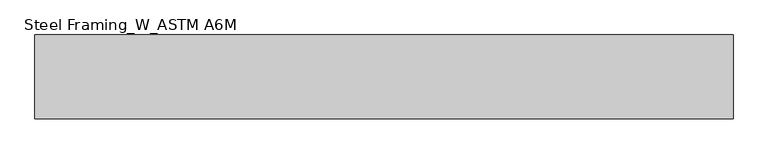
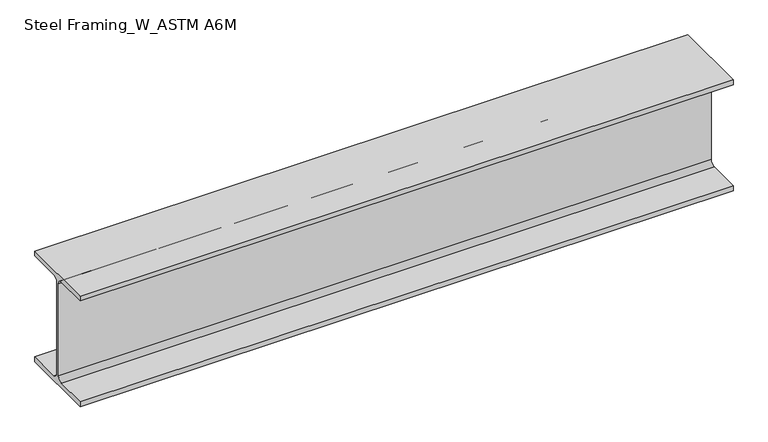
"""IFC4 building model written with IfcOpenShell, lengths in millimetres: beam geometry, Steel Framing_W_ASTM A6M : H_SB_AR_S02_W310x60_B5."""

import ifcopenshell
import ifcopenshell.guid

model = None  # the IFC model being written
_history = None  # IfcOwnerHistory: only IFC2X3 demands one
_inside = {}  # id of a spatial element -> (the spatial element, [elements in it])
_under = {}  # id of a project, library or spatial element -> (it, [spatial elements below it])
_declared = {}  # id of a project -> (the project, [libraries it declares])
_typed = {}  # id of a type object -> (the type object, [elements of that type])
_made_of = {}  # id of a material, layer set ... -> (it, [elements and type objects made of it])


def new_model(schema):
    """Start an empty IFC model of exactly this schema.

    Asked for "IFC4X3", IfcOpenShell would pick the latest addendum, in which some entities
    have other attributes; the version numbers below select the first issue.
    IFC2X3 requires an IfcOwnerHistory on every rooted entity: one is made here for all.
    """
    global model, _history
    if schema == "IFC4X3":
        model = ifcopenshell.file(schema_version=(4, 3, 0, 0))
    else:
        model = ifcopenshell.file(schema=schema)
    _inside.clear()
    _under.clear()
    _declared.clear()
    _typed.clear()
    _made_of.clear()
    _history = None
    if model.schema == "IFC2X3":
        org = make("IfcOrganization", Name="unknown")
        user = make(
            "IfcPersonAndOrganization",
            ThePerson=make("IfcPerson", FamilyName="unknown"),
            TheOrganization=org,
        )
        app = make(
            "IfcApplication",
            ApplicationDeveloper=org,
            Version="unknown",
            ApplicationFullName="unknown",
            ApplicationIdentifier="unknown",
        )
        _history = make(
            "IfcOwnerHistory",
            OwningUser=user,
            OwningApplication=app,
            ChangeAction="ADDED",
            CreationDate=0,
        )
    return model


def make(cls, **values):
    """One entity of the class cls with the attributes given. An attribute that is None is left unset."""
    return model.create_entity(
        cls, **{name: value for name, value in values.items() if value is not None}
    )


def rooted(cls, **values):
    """An entity with a GlobalId (a new one), such as an element, a storey or a relation."""
    return make(cls, GlobalId=ifcopenshell.guid.new(), OwnerHistory=_history, **values)


def si_unit(unit_type, name, prefix=None):
    """IfcSIUnit, for example si_unit("LENGTHUNIT", "METRE", prefix="MILLI")."""
    return make("IfcSIUnit", UnitType=unit_type, Prefix=prefix, Name=name)


def assignment(units):
    """IfcUnitAssignment: the units of a project."""
    return None if units is None else make("IfcUnitAssignment", Units=units)


def point(xyz):
    """IfcCartesianPoint."""
    return None if xyz is None else make("IfcCartesianPoint", Coordinates=xyz)


def direction(xyz):
    """IfcDirection."""
    return None if xyz is None else make("IfcDirection", DirectionRatios=xyz)


def frame(location, z_axis=None, x_axis=None):
    """IfcAxis2Placement3D, a coordinate frame: its origin and axes. An axis left out is left unset."""
    return make(
        "IfcAxis2Placement3D",
        Location=point(location),
        Axis=direction(z_axis),
        RefDirection=direction(x_axis),
    )


def frame_2d(location, x_axis=None):
    """IfcAxis2Placement2D, a coordinate frame in the plane: its origin and x axis."""
    return make(
        "IfcAxis2Placement2D", Location=point(location), RefDirection=direction(x_axis)
    )


def origin():
    """The frame at (0, 0, 0) with its axes left unset."""
    return frame((0.0, 0.0, 0.0))


def place(relative_to, where):
    """IfcLocalPlacement: puts the frame where relative to a parent placement (None: the world)."""
    return make(
        "IfcLocalPlacement", PlacementRelTo=relative_to, RelativePlacement=where
    )


def context(
    kind, dimensions, precision=None, world=None, true_north=None, identifier=None
):
    """IfcGeometricRepresentationContext, for example the 3D "Model" context."""
    return make(
        "IfcGeometricRepresentationContext",
        ContextIdentifier=identifier,
        ContextType=kind,
        CoordinateSpaceDimension=dimensions,
        Precision=precision,
        WorldCoordinateSystem=world,
        TrueNorth=true_north,
    )


def project(units=None, contexts=None):
    """IfcProject with its units and contexts."""
    return rooted(
        "IfcProject",
        Name="project",
        RepresentationContexts=contexts,
        UnitsInContext=assignment(units),
    )


def spatial(cls, under=None, at=None, **own):
    """A site, building, storey or space (cls), placed at a placement, below another one or the project."""
    s = rooted(cls, ObjectPlacement=at, **own)
    if under is not None:
        _under.setdefault(under.id(), (under, []))[1].append(s)
    return s


def polyline(points):
    """IfcPolyline through the points."""
    return make("IfcPolyline", Points=[point(p) for p in points])


def circle_curve(where, radius):
    """IfcCircle in the frame where."""
    return make("IfcCircle", Position=where, Radius=radius)


def trimmed(basis, trim1, trim2, sense, master):
    """IfcTrimmedCurve: the piece of a basis curve between two trims."""
    return make(
        "IfcTrimmedCurve",
        BasisCurve=basis,
        Trim1=trim1,
        Trim2=trim2,
        SenseAgreement=sense,
        MasterRepresentation=master,
    )


def segment(curve, same_sense, transition):
    """IfcCompositeCurveSegment."""
    return make(
        "IfcCompositeCurveSegment",
        Transition=transition,
        SameSense=same_sense,
        ParentCurve=curve,
    )


def composite_curve(segments, self_intersect=None):
    """IfcCompositeCurve: segments joined end to end."""
    return make("IfcCompositeCurve", Segments=segments, SelfIntersect=self_intersect)


def outline(outer, holes=None, kind="AREA"):
    """IfcArbitraryClosedProfileDef: a profile drawn as a closed curve; with holes, ...WithVoids."""
    if holes is None:
        return make("IfcArbitraryClosedProfileDef", ProfileType=kind, OuterCurve=outer)
    return make(
        "IfcArbitraryProfileDefWithVoids",
        ProfileType=kind,
        OuterCurve=outer,
        InnerCurves=holes,
    )


def extrude(swept, where, along, depth):
    """IfcExtrudedAreaSolid: the profile swept, set in the frame where, extruded along a direction by depth."""
    return make(
        "IfcExtrudedAreaSolid",
        SweptArea=swept,
        Position=where,
        ExtrudedDirection=direction(along),
        Depth=depth,
    )


def shape(context_of_items, identifier, shape_type, items):
    """IfcShapeRepresentation: the items that make up one representation, for example the "Body"."""
    return make(
        "IfcShapeRepresentation",
        ContextOfItems=context_of_items,
        RepresentationIdentifier=identifier,
        RepresentationType=shape_type,
        Items=items,
    )


def source(mapping_origin, context_of_items, identifier, shape_type, items):
    """IfcRepresentationMap: a shape defined once, which mapped items show again and again."""
    return make(
        "IfcRepresentationMap",
        MappingOrigin=mapping_origin,
        MappedRepresentation=shape(context_of_items, identifier, shape_type, items),
    )


def transform(
    local_origin,
    x_axis=None,
    y_axis=None,
    z_axis=None,
    scale=None,
    scale2=None,
    scale3=None,
    uniform=True,
):
    """IfcCartesianTransformationOperator3D, or its non-uniform kind. x_axis, y_axis, z_axis: its Axis1, 2, 3."""
    if uniform:
        return make(
            "IfcCartesianTransformationOperator3D",
            Axis1=direction(x_axis),
            Axis2=direction(y_axis),
            LocalOrigin=point(local_origin),
            Scale=scale,
            Axis3=direction(z_axis),
        )
    return make(
        "IfcCartesianTransformationOperator3DnonUniform",
        Axis1=direction(x_axis),
        Axis2=direction(y_axis),
        LocalOrigin=point(local_origin),
        Scale=scale,
        Axis3=direction(z_axis),
        Scale2=scale2,
        Scale3=scale3,
    )


def mapped(mapping_source, mapping_target):
    """IfcMappedItem: shows the shape of a source again, moved by a transform."""
    return make(
        "IfcMappedItem", MappingSource=mapping_source, MappingTarget=mapping_target
    )


def made_of(thing, what):
    """Note that an element or type object is made of a material, layer set ...; save() writes the relation."""
    if what is not None:
        _made_of.setdefault(what.id(), (what, []))[1].append(thing)
    return thing


def element(
    cls,
    number,
    at=None,
    inside=None,
    cuts=None,
    type_object=None,
    material=None,
    context=None,
    identifier="Body",
    shape_type=None,
    held_by="IfcProductDefinitionShape",
    body=None,
    shapes=None,
    **own,
):
    """One element of the class cls, such as IfcWall. Its Tag is "e" and its number.

    at: its placement. inside: the storey or other place that contains it. cuts: it is an
    opening in that element (IfcRelVoidsElement). A single representation is given by context,
    identifier, shape_type and body (its items); several are given by shapes. held_by: the class
    of the entity that holds the representations. save() writes the other relations.
    """
    e = rooted(cls, Tag="e%d" % number, ObjectPlacement=at, **own)
    if body is not None:
        shapes = [shape(context, identifier, shape_type, body)]
    if shapes is not None:
        e.Representation = make(held_by, Representations=shapes)
    if inside is not None:
        _inside.setdefault(inside.id(), (inside, []))[1].append(e)
    if cuts is not None:
        rooted(
            "IfcRelVoidsElement", RelatingBuildingElement=cuts, RelatedOpeningElement=e
        )
    if type_object is not None:
        _typed.setdefault(type_object.id(), (type_object, []))[1].append(e)
    return made_of(e, material)


def aggregate(whole, parts):
    """IfcRelAggregates: a whole, such as a stair, and the parts it consists of."""
    return rooted("IfcRelAggregates", RelatingObject=whole, RelatedObjects=parts)


def save(model, path):
    """Write the relations noted so far, then the file.

    IfcRelAggregates (storeys below a building ...), IfcRelContainedInSpatialStructure (elements
    in a storey), IfcRelDefinesByType, IfcRelAssociatesMaterial and IfcRelDeclares: one each for
    every whole, place, type object, material and project.
    """
    for whole, parts in _under.values():
        aggregate(whole, parts)
    for where, things in _inside.values():
        rooted(
            "IfcRelContainedInSpatialStructure",
            RelatedElements=things,
            RelatingStructure=where,
        )
    for kind, things in _typed.values():
        rooted("IfcRelDefinesByType", RelatedObjects=things, RelatingType=kind)
    for what, things in _made_of.values():
        rooted("IfcRelAssociatesMaterial", RelatedObjects=things, RelatingMaterial=what)
    for by, libraries in _declared.values():
        rooted("IfcRelDeclares", RelatingContext=by, RelatedDefinitions=libraries)
    model.write(path)


def steel_framing_w_astm_a6m_b2783e68(model_context):
    return source(origin(), model_context, "Body", "SweptSolid", [
        extrude(outline(composite_curve([segment(polyline([(101.5, -137.9), (101.5, -151.0), (-101.5, -151.0), (-101.5, -137.9), (-16.545, -137.9)]), True, "CONTINUOUS"), segment(trimmed(circle_curve(frame_2d((-16.545, -125.1)), 12.8), [point((-16.545, -137.9))], [point((-3.745, -125.1))], True, "CARTESIAN"), True, "CONTINUOUS"), segment(polyline([(-3.745, -125.1), (-3.745, 125.1)]), True, "CONTINUOUS"), segment(trimmed(circle_curve(frame_2d((-16.545, 125.1)), 12.8), [point((-3.745, 125.1))], [point((-16.545, 137.9))], True, "CARTESIAN"), True, "CONTINUOUS"), segment(polyline([(-16.545, 137.9), (-101.5, 137.9), (-101.5, 151.0), (101.5, 151.0), (101.5, 137.9), (16.545, 137.9)]), True, "CONTINUOUS"), segment(trimmed(circle_curve(frame_2d((16.545, 125.1)), 12.8), [point((16.545, 137.9))], [point((3.745, 125.1))], True, "CARTESIAN"), True, "CONTINUOUS"), segment(polyline([(3.745, 125.1), (3.745, -125.1)]), True, "CONTINUOUS"), segment(trimmed(circle_curve(frame_2d((16.545, -125.1)), 12.8), [point((3.745, -125.1))], [point((16.545, -137.9))], True, "CARTESIAN"), True, "CONTINUOUS"), segment(polyline([(16.545, -137.9), (101.5, -137.9)]), True, "CONTINUOUS")], self_intersect=False)), frame((-951.5, 0.0, 0.0), z_axis=(1.0, 0.0, 0.0), x_axis=(0.0, 1.0, 0.0)), (0.0, 0.0, 1.0), 1686.8),
    ])


if __name__ == "__main__":
    model = new_model("IFC4")
    model_context = context("Model", 3, world=origin())
    ifc_project = project(units=[si_unit("LENGTHUNIT", "METRE", prefix="MILLI")], contexts=[model_context])
    site = spatial("IfcSite", under=ifc_project)
    building = spatial("IfcBuilding", under=site)
    placement = place(None, origin())
    steel_framing_w_astm_a6m_shape = steel_framing_w_astm_a6m_b2783e68(model_context)
    element("IfcBeam", 1, ObjectType="Steel Framing_W_ASTM A6M : H_SB_AR_S02_W310x60_B5", at=placement, inside=building, context=model_context, shape_type="MappedRepresentation", body=[
        mapped(steel_framing_w_astm_a6m_shape, transform((0.0, 0.0, 0.0), x_axis=(1.0, 0.0, 0.0), y_axis=(0.0, 1.0, 0.0), z_axis=(0.0, 0.0, 1.0))),
    ])
    save(model, "model.ifc")

# Revit data of these elements
# Type "Steel Framing_W_ASTM A6M : H_SB_AR_S02_W310x60_B5"
#   Type Mark = "B5"
#   Section Name Key = "W12x40"
#   Width = 20.3 cm
#   Web Thickness = 0.749 cm
#   Web Fillet = 1.28 cm
#   Warping Constant = 387000.0 cm⁶
#   Torsional Moment of Inertia = 37.70 cm⁴
#   Section Area = 75.5 cm²
#   Plastic Modulus weak axis = 275.0 cm³
#   Plastic Modulus strong axis = 934.0 cm³
#   Perimeter = 1.38 m²/m
#   Nominal Weight = 60.00 kgf/m
#   Moment of Inertia weak axis = 1840.00 cm⁴
#   Moment of Inertia strong axis = 12800.00 cm⁴
#   Height = 30.2 cm
#   Flange Thickness = 1.31 cm
#   Elastic Modulus weak axis = 180.0 cm³
#   Elastic Modulus strong axis = 844.0 cm³
#   Centroid Vertical = 15.1 cm
#   Centroid Horizontal = 10.15 cm
#   Length [instance default] = 1500 mm
#   Structural Material [instance default] = Steel, 45-345
#   Bolt Spacing = 0
#   Assembly Code = ""
# Element 1 (IfcBeam, "Steel Framing_W_ASTM A6M : H_SB_AR_S02_W310x60_B5")
#   Materials on its faces: "Steel, 45-345"
# Materials
#   "Steel, 45-345": class "Metal", colour RGB 189 187 185, transparency 0, Description = "Steel 345 MPa", Cost = 0
